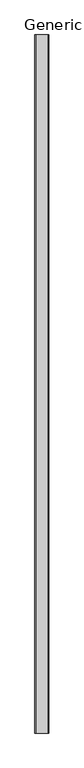
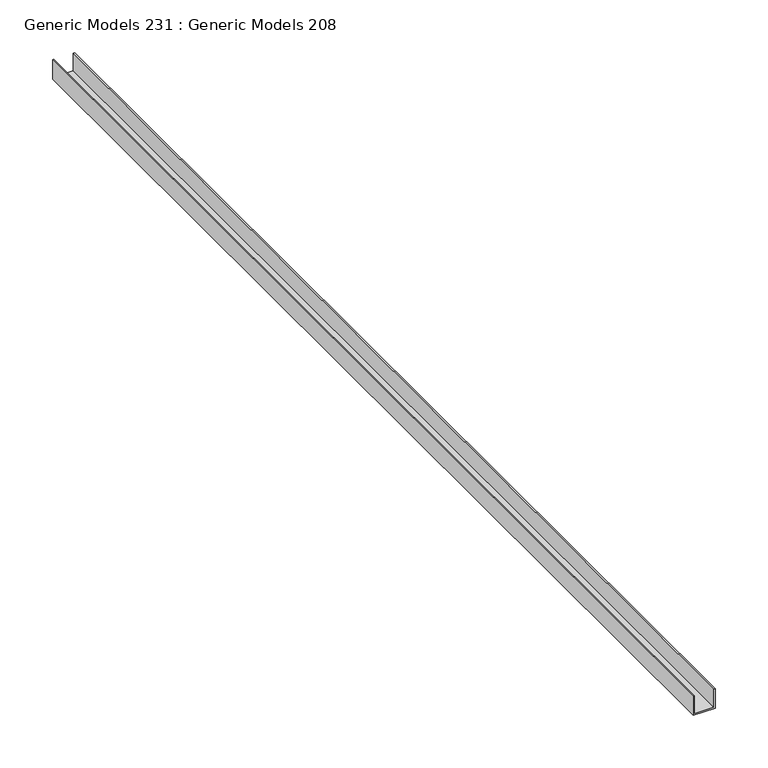
"""IFC4 building model written with IfcOpenShell, lengths in millimetres: proxy geometry, Generic Models 231 : Generic Models 208."""

from ifc_helpers import new_model, si_unit, frame, origin, place, context, project, spatial, polyline, outline, extrude, source, transform, mapped, element, save


def generic_models_231_generic_models_208_0d918d4e(model_context):
    return source(origin(), model_context, "Body", "SweptSolid", [
        extrude(outline(polyline([(2151.7306366, 54406.9921676), (2130.9815912, 54406.9921676), (2130.9815912, 54385.6357481), (2151.7306366, 54385.6357481), (2151.7306366, 54384.0482481), (2129.3940912, 54384.0482481), (2129.3940912, 54408.5796676), (2151.7306366, 54408.5796676), (2151.7306366, 54406.9921676)])), frame((0.0, -228.7033818, 0.0), z_axis=(0.0, 1.0, 0.0), x_axis=(0.0, 0.0, 1.0)), (0.0, 0.0, 1.0), 1219.2),
    ])


if __name__ == "__main__":
    model = new_model("IFC4")
    model_context = context("Model", 3, world=origin())
    ifc_project = project(units=[si_unit("LENGTHUNIT", "METRE", prefix="MILLI")], contexts=[model_context])
    site = spatial("IfcSite", under=ifc_project)
    building = spatial("IfcBuilding", under=site)
    placement = place(None, origin())
    generic_models_231_generic_models_208_shape = generic_models_231_generic_models_208_0d918d4e(model_context)
    element("IfcBuildingElementProxy", 1, Name="Generic Models 231 : Generic Models 208", ObjectType="Generic Models 231 : Generic Models 208", at=placement, inside=building, context=model_context, shape_type="MappedRepresentation", body=[
        mapped(generic_models_231_generic_models_208_shape, transform((0.0, 0.0, 0.0), x_axis=(1.0, 0.0, 0.0), y_axis=(0.0, 1.0, 0.0), z_axis=(0.0, 0.0, 1.0))),
    ])
    save(model, "model.ifc")
